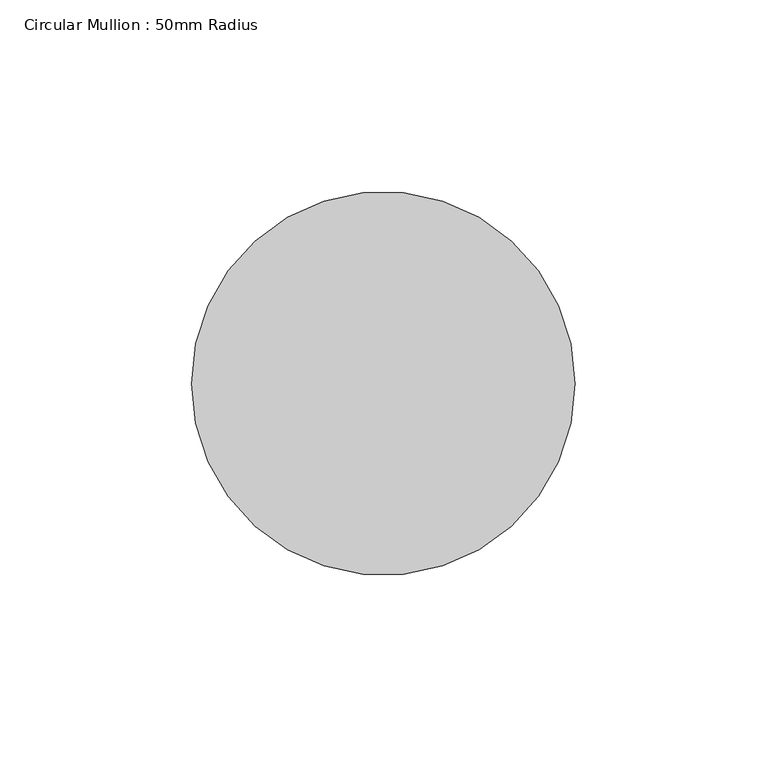
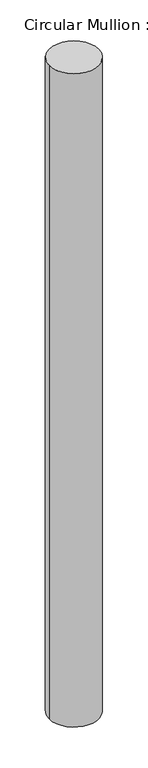
"""IFC4 building model written with IfcOpenShell, lengths in millimetres: member geometry, Circular Mullion : 50mm Radius."""

from ifc_helpers import new_model, si_unit, point, frame, origin, origin_2d, place, context, project, spatial, circle_curve, trimmed, segment, composite_curve, outline, extrude, source, transform, mapped, element, save


def circular_mullion_50mm_radius_f3ca41e8(model_context):
    return source(origin(), model_context, "Body", "SweptSolid", [
        extrude(outline(composite_curve([segment(trimmed(circle_curve(origin_2d(), 50.0), [point((50.0, 0.0))], [point((-50.0, 0.0))], False, "CARTESIAN"), True, "CONTINUOUS"), segment(trimmed(circle_curve(origin_2d(), 50.0), [point((-50.0, 0.0))], [point((50.0, 0.0))], False, "CARTESIAN"), True, "CONTINUOUS")], self_intersect=False)), frame((0.0, 0.0, -1397.3292864), z_axis=(0.0, 0.0, 1.0), x_axis=(1.0, 0.0, 0.0)), (0.0, 0.0, 1.0), 1397.3292864),
    ])


if __name__ == "__main__":
    model = new_model("IFC4")
    model_context = context("Model", 3, world=origin())
    ifc_project = project(units=[si_unit("LENGTHUNIT", "METRE", prefix="MILLI")], contexts=[model_context])
    site = spatial("IfcSite", under=ifc_project)
    building = spatial("IfcBuilding", under=site)
    placement = place(None, origin())
    circular_mullion_50mm_radius_shape = circular_mullion_50mm_radius_f3ca41e8(model_context)
    element("IfcMember", 1, ObjectType="Circular Mullion : 50mm Radius", at=placement, inside=building, context=model_context, shape_type="MappedRepresentation", body=[
        mapped(circular_mullion_50mm_radius_shape, transform((0.0, 0.0, 0.0), x_axis=(1.0, 0.0, 0.0), y_axis=(0.0, 1.0, 0.0), z_axis=(0.0, 0.0, 1.0))),
    ])
    save(model, "model.ifc")

# Revit data of these elements
# Type "Circular Mullion : 50mm Radius"
#   built-in parameter 1007350 = 0.164042 (stored number, unit not read)
# Element 1 (IfcMember, "Circular Mullion : 50mm Radius")
#   Materials on its faces: "Aluminium"
# Materials
#   "Aluminium": class "Metal", colour RGB 247 247 247, transparency 0, Description = "Aluminium 6061", Cost = 0
